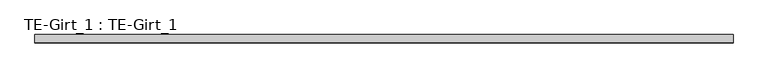
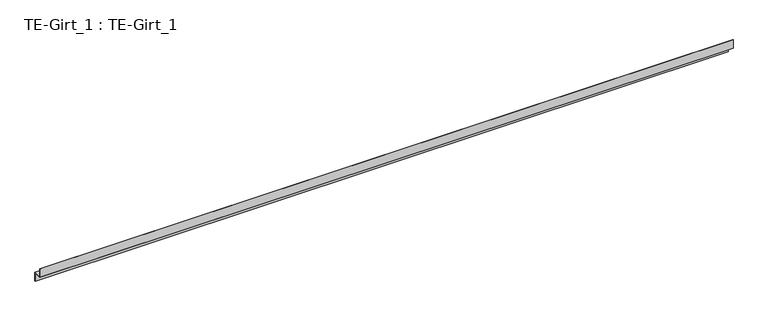
"""IFC4 building model written with IfcOpenShell, lengths in millimetres: proxy geometry, TE-Girt_1 : TE-Girt_1."""

import ifcopenshell
import ifcopenshell.guid

model = None  # the IFC model being written
_history = None  # IfcOwnerHistory: only IFC2X3 demands one
_inside = {}  # id of a spatial element -> (the spatial element, [elements in it])
_under = {}  # id of a project, library or spatial element -> (it, [spatial elements below it])
_declared = {}  # id of a project -> (the project, [libraries it declares])
_typed = {}  # id of a type object -> (the type object, [elements of that type])
_made_of = {}  # id of a material, layer set ... -> (it, [elements and type objects made of it])


def new_model(schema):
    """Start an empty IFC model of exactly this schema.

    Asked for "IFC4X3", IfcOpenShell would pick the latest addendum, in which some entities
    have other attributes; the version numbers below select the first issue.
    IFC2X3 requires an IfcOwnerHistory on every rooted entity: one is made here for all.
    """
    global model, _history
    if schema == "IFC4X3":
        model = ifcopenshell.file(schema_version=(4, 3, 0, 0))
    else:
        model = ifcopenshell.file(schema=schema)
    _inside.clear()
    _under.clear()
    _declared.clear()
    _typed.clear()
    _made_of.clear()
    _history = None
    if model.schema == "IFC2X3":
        org = make("IfcOrganization", Name="unknown")
        user = make(
            "IfcPersonAndOrganization",
            ThePerson=make("IfcPerson", FamilyName="unknown"),
            TheOrganization=org,
        )
        app = make(
            "IfcApplication",
            ApplicationDeveloper=org,
            Version="unknown",
            ApplicationFullName="unknown",
            ApplicationIdentifier="unknown",
        )
        _history = make(
            "IfcOwnerHistory",
            OwningUser=user,
            OwningApplication=app,
            ChangeAction="ADDED",
            CreationDate=0,
        )
    return model


def make(cls, **values):
    """One entity of the class cls with the attributes given. An attribute that is None is left unset."""
    return model.create_entity(
        cls, **{name: value for name, value in values.items() if value is not None}
    )


def rooted(cls, **values):
    """An entity with a GlobalId (a new one), such as an element, a storey or a relation."""
    return make(cls, GlobalId=ifcopenshell.guid.new(), OwnerHistory=_history, **values)


def si_unit(unit_type, name, prefix=None):
    """IfcSIUnit, for example si_unit("LENGTHUNIT", "METRE", prefix="MILLI")."""
    return make("IfcSIUnit", UnitType=unit_type, Prefix=prefix, Name=name)


def assignment(units):
    """IfcUnitAssignment: the units of a project."""
    return None if units is None else make("IfcUnitAssignment", Units=units)


def point(xyz):
    """IfcCartesianPoint."""
    return None if xyz is None else make("IfcCartesianPoint", Coordinates=xyz)


def direction(xyz):
    """IfcDirection."""
    return None if xyz is None else make("IfcDirection", DirectionRatios=xyz)


def frame(location, z_axis=None, x_axis=None):
    """IfcAxis2Placement3D, a coordinate frame: its origin and axes. An axis left out is left unset."""
    return make(
        "IfcAxis2Placement3D",
        Location=point(location),
        Axis=direction(z_axis),
        RefDirection=direction(x_axis),
    )


def origin():
    """The frame at (0, 0, 0) with its axes left unset."""
    return frame((0.0, 0.0, 0.0))


def place(relative_to, where):
    """IfcLocalPlacement: puts the frame where relative to a parent placement (None: the world)."""
    return make(
        "IfcLocalPlacement", PlacementRelTo=relative_to, RelativePlacement=where
    )


def context(
    kind, dimensions, precision=None, world=None, true_north=None, identifier=None
):
    """IfcGeometricRepresentationContext, for example the 3D "Model" context."""
    return make(
        "IfcGeometricRepresentationContext",
        ContextIdentifier=identifier,
        ContextType=kind,
        CoordinateSpaceDimension=dimensions,
        Precision=precision,
        WorldCoordinateSystem=world,
        TrueNorth=true_north,
    )


def project(units=None, contexts=None):
    """IfcProject with its units and contexts."""
    return rooted(
        "IfcProject",
        Name="project",
        RepresentationContexts=contexts,
        UnitsInContext=assignment(units),
    )


def spatial(cls, under=None, at=None, **own):
    """A site, building, storey or space (cls), placed at a placement, below another one or the project."""
    s = rooted(cls, ObjectPlacement=at, **own)
    if under is not None:
        _under.setdefault(under.id(), (under, []))[1].append(s)
    return s


def polyline(points):
    """IfcPolyline through the points."""
    return make("IfcPolyline", Points=[point(p) for p in points])


def outline(outer, holes=None, kind="AREA"):
    """IfcArbitraryClosedProfileDef: a profile drawn as a closed curve; with holes, ...WithVoids."""
    if holes is None:
        return make("IfcArbitraryClosedProfileDef", ProfileType=kind, OuterCurve=outer)
    return make(
        "IfcArbitraryProfileDefWithVoids",
        ProfileType=kind,
        OuterCurve=outer,
        InnerCurves=holes,
    )


def extrude(swept, where, along, depth):
    """IfcExtrudedAreaSolid: the profile swept, set in the frame where, extruded along a direction by depth."""
    return make(
        "IfcExtrudedAreaSolid",
        SweptArea=swept,
        Position=where,
        ExtrudedDirection=direction(along),
        Depth=depth,
    )


def shape(context_of_items, identifier, shape_type, items):
    """IfcShapeRepresentation: the items that make up one representation, for example the "Body"."""
    return make(
        "IfcShapeRepresentation",
        ContextOfItems=context_of_items,
        RepresentationIdentifier=identifier,
        RepresentationType=shape_type,
        Items=items,
    )


def source(mapping_origin, context_of_items, identifier, shape_type, items):
    """IfcRepresentationMap: a shape defined once, which mapped items show again and again."""
    return make(
        "IfcRepresentationMap",
        MappingOrigin=mapping_origin,
        MappedRepresentation=shape(context_of_items, identifier, shape_type, items),
    )


def transform(
    local_origin,
    x_axis=None,
    y_axis=None,
    z_axis=None,
    scale=None,
    scale2=None,
    scale3=None,
    uniform=True,
):
    """IfcCartesianTransformationOperator3D, or its non-uniform kind. x_axis, y_axis, z_axis: its Axis1, 2, 3."""
    if uniform:
        return make(
            "IfcCartesianTransformationOperator3D",
            Axis1=direction(x_axis),
            Axis2=direction(y_axis),
            LocalOrigin=point(local_origin),
            Scale=scale,
            Axis3=direction(z_axis),
        )
    return make(
        "IfcCartesianTransformationOperator3DnonUniform",
        Axis1=direction(x_axis),
        Axis2=direction(y_axis),
        LocalOrigin=point(local_origin),
        Scale=scale,
        Axis3=direction(z_axis),
        Scale2=scale2,
        Scale3=scale3,
    )


def mapped(mapping_source, mapping_target):
    """IfcMappedItem: shows the shape of a source again, moved by a transform."""
    return make(
        "IfcMappedItem", MappingSource=mapping_source, MappingTarget=mapping_target
    )


def made_of(thing, what):
    """Note that an element or type object is made of a material, layer set ...; save() writes the relation."""
    if what is not None:
        _made_of.setdefault(what.id(), (what, []))[1].append(thing)
    return thing


def element(
    cls,
    number,
    at=None,
    inside=None,
    cuts=None,
    type_object=None,
    material=None,
    context=None,
    identifier="Body",
    shape_type=None,
    held_by="IfcProductDefinitionShape",
    body=None,
    shapes=None,
    **own,
):
    """One element of the class cls, such as IfcWall. Its Tag is "e" and its number.

    at: its placement. inside: the storey or other place that contains it. cuts: it is an
    opening in that element (IfcRelVoidsElement). A single representation is given by context,
    identifier, shape_type and body (its items); several are given by shapes. held_by: the class
    of the entity that holds the representations. save() writes the other relations.
    """
    e = rooted(cls, Tag="e%d" % number, ObjectPlacement=at, **own)
    if body is not None:
        shapes = [shape(context, identifier, shape_type, body)]
    if shapes is not None:
        e.Representation = make(held_by, Representations=shapes)
    if inside is not None:
        _inside.setdefault(inside.id(), (inside, []))[1].append(e)
    if cuts is not None:
        rooted(
            "IfcRelVoidsElement", RelatingBuildingElement=cuts, RelatedOpeningElement=e
        )
    if type_object is not None:
        _typed.setdefault(type_object.id(), (type_object, []))[1].append(e)
    return made_of(e, material)


def aggregate(whole, parts):
    """IfcRelAggregates: a whole, such as a stair, and the parts it consists of."""
    return rooted("IfcRelAggregates", RelatingObject=whole, RelatedObjects=parts)


def save(model, path):
    """Write the relations noted so far, then the file.

    IfcRelAggregates (storeys below a building ...), IfcRelContainedInSpatialStructure (elements
    in a storey), IfcRelDefinesByType, IfcRelAssociatesMaterial and IfcRelDeclares: one each for
    every whole, place, type object, material and project.
    """
    for whole, parts in _under.values():
        aggregate(whole, parts)
    for where, things in _inside.values():
        rooted(
            "IfcRelContainedInSpatialStructure",
            RelatedElements=things,
            RelatingStructure=where,
        )
    for kind, things in _typed.values():
        rooted("IfcRelDefinesByType", RelatedObjects=things, RelatingType=kind)
    for what, things in _made_of.values():
        rooted("IfcRelAssociatesMaterial", RelatedObjects=things, RelatingMaterial=what)
    for by, libraries in _declared.values():
        rooted("IfcRelDeclares", RelatingContext=by, RelatedDefinitions=libraries)
    model.write(path)


def te_girt_1_te_girt_1_0389d321(model_context):
    return source(origin(), model_context, "Body", "SweptSolid", [
        extrude(outline(polyline([(-531639.2163841, 844.55), (-531639.2163841, 806.45), (-531640.1093528, 806.45), (-531640.1093528, 843.6570312), (-531674.1249348, 843.6570312), (-531674.1249348, 881.7570312), (-531673.231966, 881.7570312), (-531673.231966, 844.55), (-531639.2163841, 844.55)])), frame((587397.6434739, 0.0, 0.0), z_axis=(1.0, 0.0, 0.0), x_axis=(0.0, 1.0, 0.0)), (0.0, 0.0, 1.0), 2921.0),
    ])


if __name__ == "__main__":
    model = new_model("IFC4")
    model_context = context("Model", 3, world=origin())
    ifc_project = project(units=[si_unit("LENGTHUNIT", "METRE", prefix="MILLI")], contexts=[model_context])
    site = spatial("IfcSite", under=ifc_project)
    building = spatial("IfcBuilding", under=site)
    placement = place(None, origin())
    te_girt_1_te_girt_1_shape = te_girt_1_te_girt_1_0389d321(model_context)
    element("IfcBuildingElementProxy", 1, Name="TE-Girt_1 : TE-Girt_1", ObjectType="TE-Girt_1 : TE-Girt_1", at=placement, inside=building, context=model_context, shape_type="MappedRepresentation", body=[
        mapped(te_girt_1_te_girt_1_shape, transform((0.0, 0.0, 0.0), x_axis=(1.0, 0.0, 0.0), y_axis=(0.0, 1.0, 0.0), z_axis=(0.0, 0.0, 1.0))),
    ])
    save(model, "model.ifc")

# Revit data of these elements
# Element 1 (IfcBuildingElementProxy, "TE-Girt_1 : TE-Girt_1")
#   Materials on its faces: "Z-FURRING, COLD-FORMED GALV."
# Materials
#   "Z-FURRING, COLD-FORMED GALV.": class "Generic", colour RGB 143 142 141, transparency 0, Cost = 0
